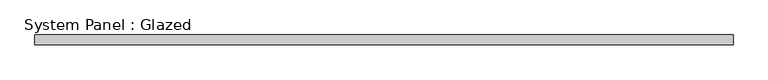
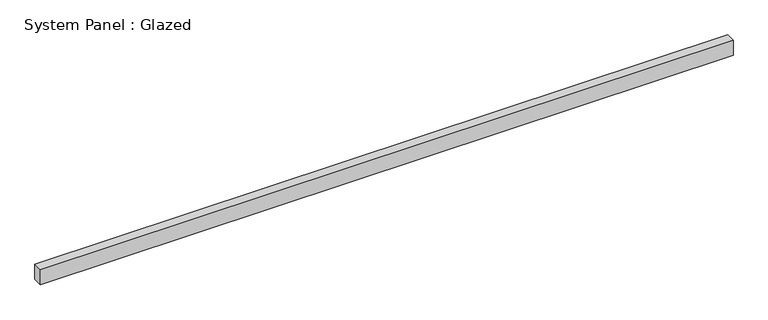
"""IFC4 building model written with IfcOpenShell, lengths in millimetres: plate geometry, System Panel : Glazed."""

import ifcopenshell
import ifcopenshell.guid

model = None  # the IFC model being written
_history = None  # IfcOwnerHistory: only IFC2X3 demands one
_inside = {}  # id of a spatial element -> (the spatial element, [elements in it])
_under = {}  # id of a project, library or spatial element -> (it, [spatial elements below it])
_declared = {}  # id of a project -> (the project, [libraries it declares])
_typed = {}  # id of a type object -> (the type object, [elements of that type])
_made_of = {}  # id of a material, layer set ... -> (it, [elements and type objects made of it])


def new_model(schema):
    """Start an empty IFC model of exactly this schema.

    Asked for "IFC4X3", IfcOpenShell would pick the latest addendum, in which some entities
    have other attributes; the version numbers below select the first issue.
    IFC2X3 requires an IfcOwnerHistory on every rooted entity: one is made here for all.
    """
    global model, _history
    if schema == "IFC4X3":
        model = ifcopenshell.file(schema_version=(4, 3, 0, 0))
    else:
        model = ifcopenshell.file(schema=schema)
    _inside.clear()
    _under.clear()
    _declared.clear()
    _typed.clear()
    _made_of.clear()
    _history = None
    if model.schema == "IFC2X3":
        org = make("IfcOrganization", Name="unknown")
        user = make(
            "IfcPersonAndOrganization",
            ThePerson=make("IfcPerson", FamilyName="unknown"),
            TheOrganization=org,
        )
        app = make(
            "IfcApplication",
            ApplicationDeveloper=org,
            Version="unknown",
            ApplicationFullName="unknown",
            ApplicationIdentifier="unknown",
        )
        _history = make(
            "IfcOwnerHistory",
            OwningUser=user,
            OwningApplication=app,
            ChangeAction="ADDED",
            CreationDate=0,
        )
    return model


def make(cls, **values):
    """One entity of the class cls with the attributes given. An attribute that is None is left unset."""
    return model.create_entity(
        cls, **{name: value for name, value in values.items() if value is not None}
    )


def rooted(cls, **values):
    """An entity with a GlobalId (a new one), such as an element, a storey or a relation."""
    return make(cls, GlobalId=ifcopenshell.guid.new(), OwnerHistory=_history, **values)


def si_unit(unit_type, name, prefix=None):
    """IfcSIUnit, for example si_unit("LENGTHUNIT", "METRE", prefix="MILLI")."""
    return make("IfcSIUnit", UnitType=unit_type, Prefix=prefix, Name=name)


def assignment(units):
    """IfcUnitAssignment: the units of a project."""
    return None if units is None else make("IfcUnitAssignment", Units=units)


def point(xyz):
    """IfcCartesianPoint."""
    return None if xyz is None else make("IfcCartesianPoint", Coordinates=xyz)


def direction(xyz):
    """IfcDirection."""
    return None if xyz is None else make("IfcDirection", DirectionRatios=xyz)


def frame(location, z_axis=None, x_axis=None):
    """IfcAxis2Placement3D, a coordinate frame: its origin and axes. An axis left out is left unset."""
    return make(
        "IfcAxis2Placement3D",
        Location=point(location),
        Axis=direction(z_axis),
        RefDirection=direction(x_axis),
    )


def origin():
    """The frame at (0, 0, 0) with its axes left unset."""
    return frame((0.0, 0.0, 0.0))


def origin_with_axes():
    """The frame at (0, 0, 0) with the z axis (0, 0, 1) and the x axis (1, 0, 0) written out."""
    return frame((0.0, 0.0, 0.0), z_axis=(0.0, 0.0, 1.0), x_axis=(1.0, 0.0, 0.0))


def place(relative_to, where):
    """IfcLocalPlacement: puts the frame where relative to a parent placement (None: the world)."""
    return make(
        "IfcLocalPlacement", PlacementRelTo=relative_to, RelativePlacement=where
    )


def context(
    kind, dimensions, precision=None, world=None, true_north=None, identifier=None
):
    """IfcGeometricRepresentationContext, for example the 3D "Model" context."""
    return make(
        "IfcGeometricRepresentationContext",
        ContextIdentifier=identifier,
        ContextType=kind,
        CoordinateSpaceDimension=dimensions,
        Precision=precision,
        WorldCoordinateSystem=world,
        TrueNorth=true_north,
    )


def project(units=None, contexts=None):
    """IfcProject with its units and contexts."""
    return rooted(
        "IfcProject",
        Name="project",
        RepresentationContexts=contexts,
        UnitsInContext=assignment(units),
    )


def spatial(cls, under=None, at=None, **own):
    """A site, building, storey or space (cls), placed at a placement, below another one or the project."""
    s = rooted(cls, ObjectPlacement=at, **own)
    if under is not None:
        _under.setdefault(under.id(), (under, []))[1].append(s)
    return s


def polyline(points):
    """IfcPolyline through the points."""
    return make("IfcPolyline", Points=[point(p) for p in points])


def outline(outer, holes=None, kind="AREA"):
    """IfcArbitraryClosedProfileDef: a profile drawn as a closed curve; with holes, ...WithVoids."""
    if holes is None:
        return make("IfcArbitraryClosedProfileDef", ProfileType=kind, OuterCurve=outer)
    return make(
        "IfcArbitraryProfileDefWithVoids",
        ProfileType=kind,
        OuterCurve=outer,
        InnerCurves=holes,
    )


def extrude(swept, where, along, depth):
    """IfcExtrudedAreaSolid: the profile swept, set in the frame where, extruded along a direction by depth."""
    return make(
        "IfcExtrudedAreaSolid",
        SweptArea=swept,
        Position=where,
        ExtrudedDirection=direction(along),
        Depth=depth,
    )


def shape(context_of_items, identifier, shape_type, items):
    """IfcShapeRepresentation: the items that make up one representation, for example the "Body"."""
    return make(
        "IfcShapeRepresentation",
        ContextOfItems=context_of_items,
        RepresentationIdentifier=identifier,
        RepresentationType=shape_type,
        Items=items,
    )


def source(mapping_origin, context_of_items, identifier, shape_type, items):
    """IfcRepresentationMap: a shape defined once, which mapped items show again and again."""
    return make(
        "IfcRepresentationMap",
        MappingOrigin=mapping_origin,
        MappedRepresentation=shape(context_of_items, identifier, shape_type, items),
    )


def transform(
    local_origin,
    x_axis=None,
    y_axis=None,
    z_axis=None,
    scale=None,
    scale2=None,
    scale3=None,
    uniform=True,
):
    """IfcCartesianTransformationOperator3D, or its non-uniform kind. x_axis, y_axis, z_axis: its Axis1, 2, 3."""
    if uniform:
        return make(
            "IfcCartesianTransformationOperator3D",
            Axis1=direction(x_axis),
            Axis2=direction(y_axis),
            LocalOrigin=point(local_origin),
            Scale=scale,
            Axis3=direction(z_axis),
        )
    return make(
        "IfcCartesianTransformationOperator3DnonUniform",
        Axis1=direction(x_axis),
        Axis2=direction(y_axis),
        LocalOrigin=point(local_origin),
        Scale=scale,
        Axis3=direction(z_axis),
        Scale2=scale2,
        Scale3=scale3,
    )


def mapped(mapping_source, mapping_target):
    """IfcMappedItem: shows the shape of a source again, moved by a transform."""
    return make(
        "IfcMappedItem", MappingSource=mapping_source, MappingTarget=mapping_target
    )


def made_of(thing, what):
    """Note that an element or type object is made of a material, layer set ...; save() writes the relation."""
    if what is not None:
        _made_of.setdefault(what.id(), (what, []))[1].append(thing)
    return thing


def element(
    cls,
    number,
    at=None,
    inside=None,
    cuts=None,
    type_object=None,
    material=None,
    context=None,
    identifier="Body",
    shape_type=None,
    held_by="IfcProductDefinitionShape",
    body=None,
    shapes=None,
    **own,
):
    """One element of the class cls, such as IfcWall. Its Tag is "e" and its number.

    at: its placement. inside: the storey or other place that contains it. cuts: it is an
    opening in that element (IfcRelVoidsElement). A single representation is given by context,
    identifier, shape_type and body (its items); several are given by shapes. held_by: the class
    of the entity that holds the representations. save() writes the other relations.
    """
    e = rooted(cls, Tag="e%d" % number, ObjectPlacement=at, **own)
    if body is not None:
        shapes = [shape(context, identifier, shape_type, body)]
    if shapes is not None:
        e.Representation = make(held_by, Representations=shapes)
    if inside is not None:
        _inside.setdefault(inside.id(), (inside, []))[1].append(e)
    if cuts is not None:
        rooted(
            "IfcRelVoidsElement", RelatingBuildingElement=cuts, RelatedOpeningElement=e
        )
    if type_object is not None:
        _typed.setdefault(type_object.id(), (type_object, []))[1].append(e)
    return made_of(e, material)


def aggregate(whole, parts):
    """IfcRelAggregates: a whole, such as a stair, and the parts it consists of."""
    return rooted("IfcRelAggregates", RelatingObject=whole, RelatedObjects=parts)


def save(model, path):
    """Write the relations noted so far, then the file.

    IfcRelAggregates (storeys below a building ...), IfcRelContainedInSpatialStructure (elements
    in a storey), IfcRelDefinesByType, IfcRelAssociatesMaterial and IfcRelDeclares: one each for
    every whole, place, type object, material and project.
    """
    for whole, parts in _under.values():
        aggregate(whole, parts)
    for where, things in _inside.values():
        rooted(
            "IfcRelContainedInSpatialStructure",
            RelatedElements=things,
            RelatingStructure=where,
        )
    for kind, things in _typed.values():
        rooted("IfcRelDefinesByType", RelatedObjects=things, RelatingType=kind)
    for what, things in _made_of.values():
        rooted("IfcRelAssociatesMaterial", RelatedObjects=things, RelatingMaterial=what)
    for by, libraries in _declared.values():
        rooted("IfcRelDeclares", RelatingContext=by, RelatedDefinitions=libraries)
    model.write(path)


def system_panel_glazed_7f82afe2(model_context):
    return source(origin(), model_context, "Body", "SweptSolid", [
        extrude(outline(polyline([(914.4, -44.45), (-914.4, -44.45), (-914.4, -19.05), (914.4, -19.05), (914.4, -44.45)])), origin_with_axes(), (0.0, 0.0, 1.0), 41.9143134),
    ])


if __name__ == "__main__":
    model = new_model("IFC4")
    model_context = context("Model", 3, world=origin())
    ifc_project = project(units=[si_unit("LENGTHUNIT", "METRE", prefix="MILLI")], contexts=[model_context])
    site = spatial("IfcSite", under=ifc_project)
    building = spatial("IfcBuilding", under=site)
    placement = place(None, origin())
    system_panel_glazed_shape = system_panel_glazed_7f82afe2(model_context)
    element("IfcPlate", 1, ObjectType="System Panel : Glazed", at=placement, inside=building, context=model_context, shape_type="MappedRepresentation", body=[
        mapped(system_panel_glazed_shape, transform((0.0, 0.0, 0.0), x_axis=(1.0, 0.0, 0.0), y_axis=(0.0, 1.0, 0.0), z_axis=(0.0, 0.0, 1.0))),
    ])
    save(model, "model.ifc")

# Revit data of these elements
# Type "System Panel : Glazed"
#   Construction Type Id = "GSP4R"
#   Analytic Construction = "1/8 in Pilkington single glazing"
#   Visual Light Transmittance = 0.9
#   Solar Heat Gain Coefficient = 0.86
#   Heat Transfer Coefficient (U) = 1.18115 BTU/(h·ft²·°F)
#   Define Thermal Properties by = 1
# Element 1 (IfcPlate, "System Panel : Glazed")
#   Materials on its faces: "Glass"
# Materials
#   "Glass": class "Glass", colour RGB 0 128 192, transparency 0.75, Description = "Soda Lime Glass", Cost = 0
